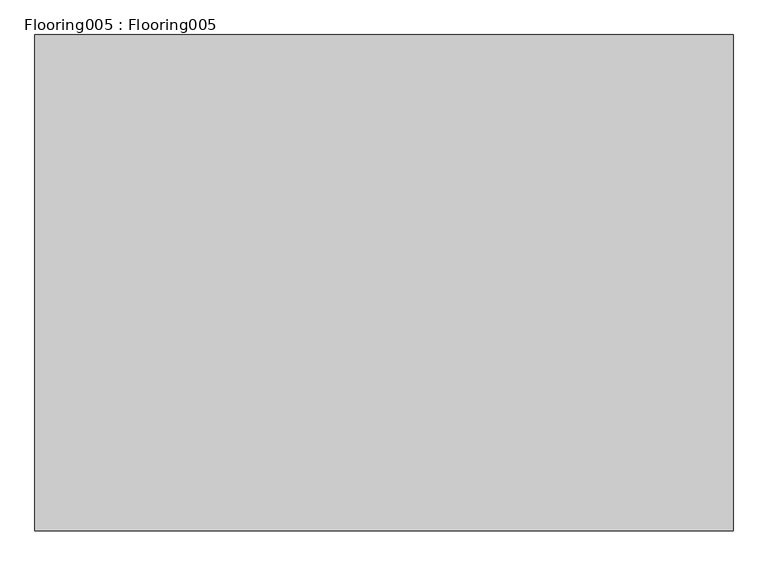
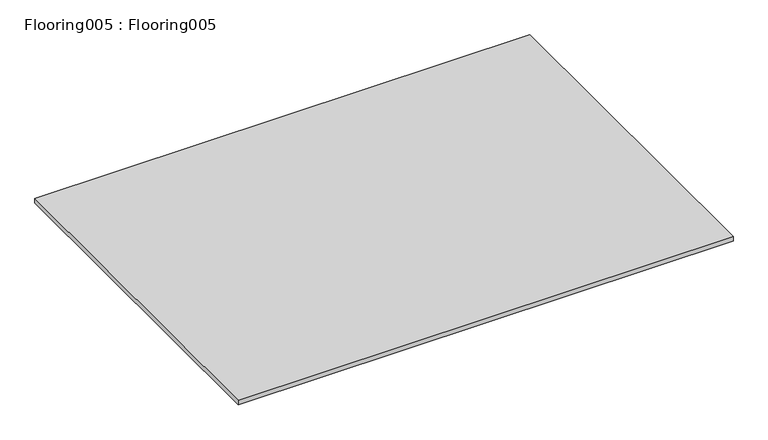
"""IFC4 building model written with IfcOpenShell, lengths in millimetres: proxy geometry, Flooring005 : Flooring005."""

from ifc_helpers import new_model, si_unit, frame, origin, place, context, project, spatial, polyline, outline, extrude, source, transform, mapped, element, save


def flooring005_flooring005_a0f2294d(model_context):
    return source(origin(), model_context, "Body", "SweptSolid", [
        extrude(outline(polyline([(12382.7678845, -4250.1925368), (12382.7678845, -2827.7925368), (14383.0178845, -2827.7925368), (14383.0178845, -4250.1925368), (12382.7678845, -4250.1925368)])), frame((0.0, 0.0, 40112.696), z_axis=(0.0, 0.0, 1.0), x_axis=(1.0, 0.0, 0.0)), (0.0, 0.0, 1.0), 19.05),
    ])


if __name__ == "__main__":
    model = new_model("IFC4")
    model_context = context("Model", 3, world=origin())
    ifc_project = project(units=[si_unit("LENGTHUNIT", "METRE", prefix="MILLI")], contexts=[model_context])
    site = spatial("IfcSite", under=ifc_project)
    building = spatial("IfcBuilding", under=site)
    placement = place(None, origin())
    flooring005_flooring005_shape = flooring005_flooring005_a0f2294d(model_context)
    element("IfcBuildingElementProxy", 1, Name="Flooring005 : Flooring005", ObjectType="Flooring005 : Flooring005", at=placement, inside=building, context=model_context, shape_type="MappedRepresentation", body=[
        mapped(flooring005_flooring005_shape, transform((0.0, 0.0, 0.0), x_axis=(1.0, 0.0, 0.0), y_axis=(0.0, 1.0, 0.0), z_axis=(0.0, 0.0, 1.0))),
    ])
    save(model, "model.ifc")

# Revit data of these elements
# Type "Flooring005 : Flooring005"
#   NameOverride = "Flooring005"
# Element 1 (IfcBuildingElementProxy, "Flooring005 : Flooring005")
#   Materials on its faces: "CDX PLYWOOD - SEE STRUCTURAL DWGS"
# Materials
#   "CDX PLYWOOD - SEE STRUCTURAL DWGS": class "Unassigned", colour RGB 177 130 114, transparency 0, Cost = 0
